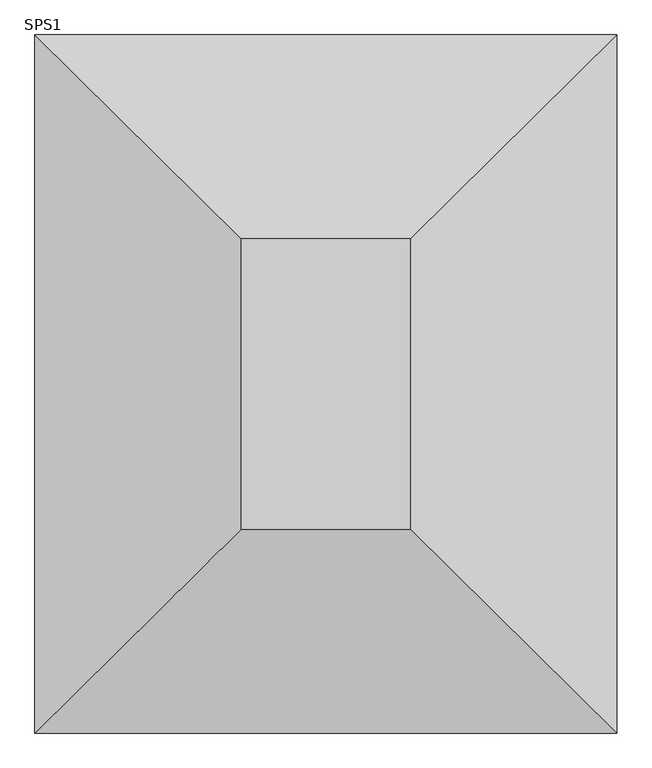
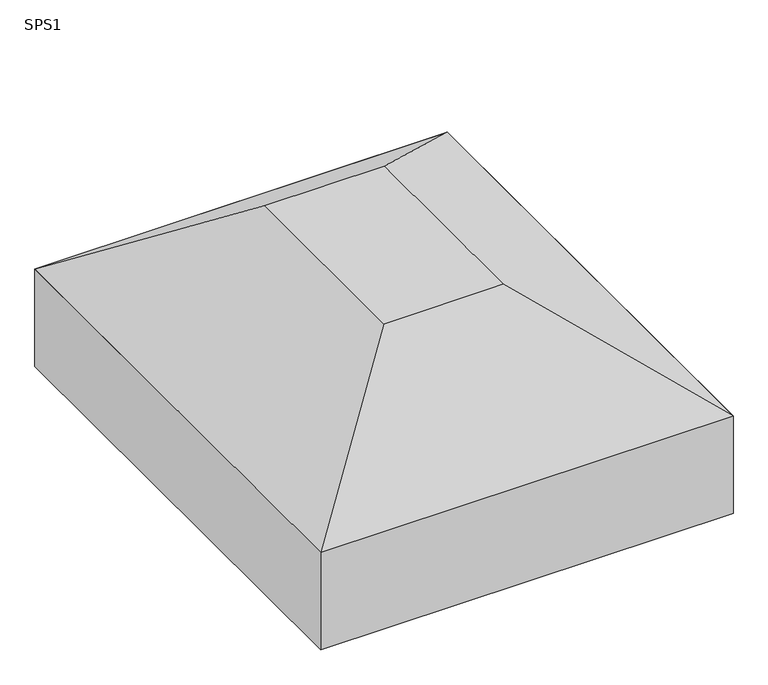
"""IFC4 building model written with IfcOpenShell, lengths in millimetres: fastener geometry, TQS - Sapata : SPS1."""

from ifc_helpers import new_model, si_unit, frame, origin, place, context, project, spatial, polyline, outline, extrude, faceted_brep, source, transform, mapped, element, save


def sps1_6b3be553(model_context):
    return source(origin(), model_context, "Body", "SolidModel", [
        faceted_brep([(-55.0, 50.0, 0.0), (-345.0, 50.0, 0.0), (-345.0, -450.0, 0.0), (-55.0, -450.0, 0.0), (300.0, 400.0, -250.0), (300.0, -800.0, -250.0), (-700.0, -800.0, -250.0), (-700.0, 400.0, -250.0)], [[[0, 1, 2, 3]], [[4, 5, 6, 7]], [[4, 7, 1, 0]], [[7, 6, 2, 1]], [[6, 5, 3, 2]], [[5, 4, 0, 3]]]),
        extrude(outline(polyline([(300.0, 400.0), (300.0, -800.0), (-700.0, -800.0), (-700.0, 400.0), (300.0, 400.0)])), frame((0.0, 0.0, -500.0), z_axis=(0.0, 0.0, 1.0), x_axis=(1.0, 0.0, 0.0)), (0.0, 0.0, 1.0), 250.0),
    ])


if __name__ == "__main__":
    model = new_model("IFC4")
    model_context = context("Model", 3, world=origin())
    ifc_project = project(units=[si_unit("LENGTHUNIT", "METRE", prefix="MILLI")], contexts=[model_context])
    site = spatial("IfcSite", under=ifc_project)
    building = spatial("IfcBuilding", under=site)
    placement = place(None, origin())
    sps1_shape = sps1_6b3be553(model_context)
    element("IfcFastener", 1, ObjectType="TQS - Sapata : SPS1", at=placement, inside=building, context=model_context, shape_type="MappedRepresentation", body=[
        mapped(sps1_shape, transform((0.0, 0.0, 0.0), x_axis=(1.0, 0.0, 0.0), y_axis=(0.0, 1.0, 0.0), z_axis=(0.0, 0.0, 1.0))),
    ])
    save(model, "model.ifc")

# Revit data of these elements
# Type "TQS - Sapata : SPS1"
#   TY = 0.50 m
#   TX = 0.29 m
#   HS = 0.50 m
#   H0 = 0.25 m
#   EXCYABS = 0.60 m
#   EXCY = 0.00 m
#   EXCXABS = 0.50 m
#   EXCX = 0.00 m
#   DIMY = 1.20 m
#   DIMX = 1.00 m
#   Material estrutural = Concreto - Concreto concretado no local
#   Width = 0
#   Length = 0
# Element 1 (IfcFastener, "TQS - Sapata : SPS1")
#   Materials on its faces: "Concreto - Concreto concretado no local"
# Materials
#   "Concreto - Concreto concretado no local": class "Concreto", colour RGB 192 192 192, transparency 0
